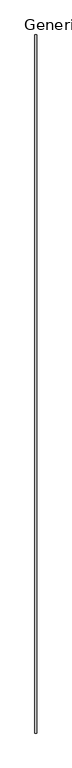
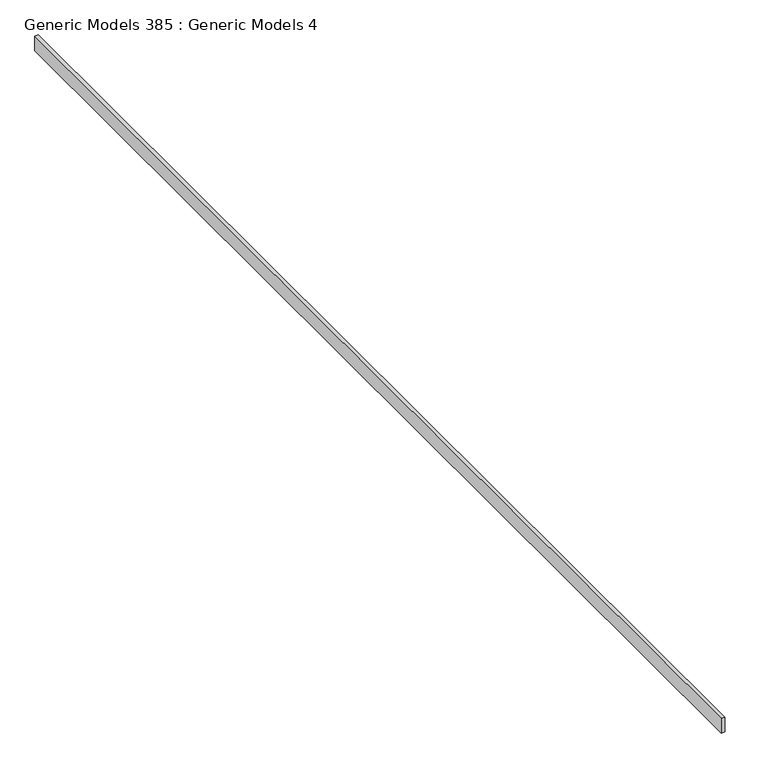
"""IFC4 building model written with IfcOpenShell, lengths in millimetres: proxy geometry, Generic Models 385 : Generic Models 4."""

import ifcopenshell
import ifcopenshell.guid

model = None  # the IFC model being written
_history = None  # IfcOwnerHistory: only IFC2X3 demands one
_inside = {}  # id of a spatial element -> (the spatial element, [elements in it])
_under = {}  # id of a project, library or spatial element -> (it, [spatial elements below it])
_declared = {}  # id of a project -> (the project, [libraries it declares])
_typed = {}  # id of a type object -> (the type object, [elements of that type])
_made_of = {}  # id of a material, layer set ... -> (it, [elements and type objects made of it])


def new_model(schema):
    """Start an empty IFC model of exactly this schema.

    Asked for "IFC4X3", IfcOpenShell would pick the latest addendum, in which some entities
    have other attributes; the version numbers below select the first issue.
    IFC2X3 requires an IfcOwnerHistory on every rooted entity: one is made here for all.
    """
    global model, _history
    if schema == "IFC4X3":
        model = ifcopenshell.file(schema_version=(4, 3, 0, 0))
    else:
        model = ifcopenshell.file(schema=schema)
    _inside.clear()
    _under.clear()
    _declared.clear()
    _typed.clear()
    _made_of.clear()
    _history = None
    if model.schema == "IFC2X3":
        org = make("IfcOrganization", Name="unknown")
        user = make(
            "IfcPersonAndOrganization",
            ThePerson=make("IfcPerson", FamilyName="unknown"),
            TheOrganization=org,
        )
        app = make(
            "IfcApplication",
            ApplicationDeveloper=org,
            Version="unknown",
            ApplicationFullName="unknown",
            ApplicationIdentifier="unknown",
        )
        _history = make(
            "IfcOwnerHistory",
            OwningUser=user,
            OwningApplication=app,
            ChangeAction="ADDED",
            CreationDate=0,
        )
    return model


def make(cls, **values):
    """One entity of the class cls with the attributes given. An attribute that is None is left unset."""
    return model.create_entity(
        cls, **{name: value for name, value in values.items() if value is not None}
    )


def rooted(cls, **values):
    """An entity with a GlobalId (a new one), such as an element, a storey or a relation."""
    return make(cls, GlobalId=ifcopenshell.guid.new(), OwnerHistory=_history, **values)


def si_unit(unit_type, name, prefix=None):
    """IfcSIUnit, for example si_unit("LENGTHUNIT", "METRE", prefix="MILLI")."""
    return make("IfcSIUnit", UnitType=unit_type, Prefix=prefix, Name=name)


def assignment(units):
    """IfcUnitAssignment: the units of a project."""
    return None if units is None else make("IfcUnitAssignment", Units=units)


def point(xyz):
    """IfcCartesianPoint."""
    return None if xyz is None else make("IfcCartesianPoint", Coordinates=xyz)


def direction(xyz):
    """IfcDirection."""
    return None if xyz is None else make("IfcDirection", DirectionRatios=xyz)


def frame(location, z_axis=None, x_axis=None):
    """IfcAxis2Placement3D, a coordinate frame: its origin and axes. An axis left out is left unset."""
    return make(
        "IfcAxis2Placement3D",
        Location=point(location),
        Axis=direction(z_axis),
        RefDirection=direction(x_axis),
    )


def origin():
    """The frame at (0, 0, 0) with its axes left unset."""
    return frame((0.0, 0.0, 0.0))


def place(relative_to, where):
    """IfcLocalPlacement: puts the frame where relative to a parent placement (None: the world)."""
    return make(
        "IfcLocalPlacement", PlacementRelTo=relative_to, RelativePlacement=where
    )


def context(
    kind, dimensions, precision=None, world=None, true_north=None, identifier=None
):
    """IfcGeometricRepresentationContext, for example the 3D "Model" context."""
    return make(
        "IfcGeometricRepresentationContext",
        ContextIdentifier=identifier,
        ContextType=kind,
        CoordinateSpaceDimension=dimensions,
        Precision=precision,
        WorldCoordinateSystem=world,
        TrueNorth=true_north,
    )


def project(units=None, contexts=None):
    """IfcProject with its units and contexts."""
    return rooted(
        "IfcProject",
        Name="project",
        RepresentationContexts=contexts,
        UnitsInContext=assignment(units),
    )


def spatial(cls, under=None, at=None, **own):
    """A site, building, storey or space (cls), placed at a placement, below another one or the project."""
    s = rooted(cls, ObjectPlacement=at, **own)
    if under is not None:
        _under.setdefault(under.id(), (under, []))[1].append(s)
    return s


def polyline(points):
    """IfcPolyline through the points."""
    return make("IfcPolyline", Points=[point(p) for p in points])


def outline(outer, holes=None, kind="AREA"):
    """IfcArbitraryClosedProfileDef: a profile drawn as a closed curve; with holes, ...WithVoids."""
    if holes is None:
        return make("IfcArbitraryClosedProfileDef", ProfileType=kind, OuterCurve=outer)
    return make(
        "IfcArbitraryProfileDefWithVoids",
        ProfileType=kind,
        OuterCurve=outer,
        InnerCurves=holes,
    )


def extrude(swept, where, along, depth):
    """IfcExtrudedAreaSolid: the profile swept, set in the frame where, extruded along a direction by depth."""
    return make(
        "IfcExtrudedAreaSolid",
        SweptArea=swept,
        Position=where,
        ExtrudedDirection=direction(along),
        Depth=depth,
    )


def shape(context_of_items, identifier, shape_type, items):
    """IfcShapeRepresentation: the items that make up one representation, for example the "Body"."""
    return make(
        "IfcShapeRepresentation",
        ContextOfItems=context_of_items,
        RepresentationIdentifier=identifier,
        RepresentationType=shape_type,
        Items=items,
    )


def source(mapping_origin, context_of_items, identifier, shape_type, items):
    """IfcRepresentationMap: a shape defined once, which mapped items show again and again."""
    return make(
        "IfcRepresentationMap",
        MappingOrigin=mapping_origin,
        MappedRepresentation=shape(context_of_items, identifier, shape_type, items),
    )


def transform(
    local_origin,
    x_axis=None,
    y_axis=None,
    z_axis=None,
    scale=None,
    scale2=None,
    scale3=None,
    uniform=True,
):
    """IfcCartesianTransformationOperator3D, or its non-uniform kind. x_axis, y_axis, z_axis: its Axis1, 2, 3."""
    if uniform:
        return make(
            "IfcCartesianTransformationOperator3D",
            Axis1=direction(x_axis),
            Axis2=direction(y_axis),
            LocalOrigin=point(local_origin),
            Scale=scale,
            Axis3=direction(z_axis),
        )
    return make(
        "IfcCartesianTransformationOperator3DnonUniform",
        Axis1=direction(x_axis),
        Axis2=direction(y_axis),
        LocalOrigin=point(local_origin),
        Scale=scale,
        Axis3=direction(z_axis),
        Scale2=scale2,
        Scale3=scale3,
    )


def mapped(mapping_source, mapping_target):
    """IfcMappedItem: shows the shape of a source again, moved by a transform."""
    return make(
        "IfcMappedItem", MappingSource=mapping_source, MappingTarget=mapping_target
    )


def made_of(thing, what):
    """Note that an element or type object is made of a material, layer set ...; save() writes the relation."""
    if what is not None:
        _made_of.setdefault(what.id(), (what, []))[1].append(thing)
    return thing


def element(
    cls,
    number,
    at=None,
    inside=None,
    cuts=None,
    type_object=None,
    material=None,
    context=None,
    identifier="Body",
    shape_type=None,
    held_by="IfcProductDefinitionShape",
    body=None,
    shapes=None,
    **own,
):
    """One element of the class cls, such as IfcWall. Its Tag is "e" and its number.

    at: its placement. inside: the storey or other place that contains it. cuts: it is an
    opening in that element (IfcRelVoidsElement). A single representation is given by context,
    identifier, shape_type and body (its items); several are given by shapes. held_by: the class
    of the entity that holds the representations. save() writes the other relations.
    """
    e = rooted(cls, Tag="e%d" % number, ObjectPlacement=at, **own)
    if body is not None:
        shapes = [shape(context, identifier, shape_type, body)]
    if shapes is not None:
        e.Representation = make(held_by, Representations=shapes)
    if inside is not None:
        _inside.setdefault(inside.id(), (inside, []))[1].append(e)
    if cuts is not None:
        rooted(
            "IfcRelVoidsElement", RelatingBuildingElement=cuts, RelatedOpeningElement=e
        )
    if type_object is not None:
        _typed.setdefault(type_object.id(), (type_object, []))[1].append(e)
    return made_of(e, material)


def aggregate(whole, parts):
    """IfcRelAggregates: a whole, such as a stair, and the parts it consists of."""
    return rooted("IfcRelAggregates", RelatingObject=whole, RelatedObjects=parts)


def save(model, path):
    """Write the relations noted so far, then the file.

    IfcRelAggregates (storeys below a building ...), IfcRelContainedInSpatialStructure (elements
    in a storey), IfcRelDefinesByType, IfcRelAssociatesMaterial and IfcRelDeclares: one each for
    every whole, place, type object, material and project.
    """
    for whole, parts in _under.values():
        aggregate(whole, parts)
    for where, things in _inside.values():
        rooted(
            "IfcRelContainedInSpatialStructure",
            RelatedElements=things,
            RelatingStructure=where,
        )
    for kind, things in _typed.values():
        rooted("IfcRelDefinesByType", RelatedObjects=things, RelatingType=kind)
    for what, things in _made_of.values():
        rooted("IfcRelAssociatesMaterial", RelatedObjects=things, RelatingMaterial=what)
    for by, libraries in _declared.values():
        rooted("IfcRelDeclares", RelatingContext=by, RelatedDefinitions=libraries)
    model.write(path)


def generic_models_385_generic_models_4_06af05cc(model_context):
    return source(origin(), model_context, "Body", "SweptSolid", [
        extrude(outline(polyline([(8346.0514146, -6864.9230338), (8327.0014146, -6864.9230338), (8327.0014146, -464.1230338), (8346.0514146, -464.1230338), (8346.0514146, -6864.9230338)])), frame((0.0, 0.0, 126250.2332283), z_axis=(0.0, 0.0, 1.0), x_axis=(1.0, 0.0, 0.0)), (0.0, 0.0, 1.0), 83.6072898),
    ])


if __name__ == "__main__":
    model = new_model("IFC4")
    model_context = context("Model", 3, world=origin())
    ifc_project = project(units=[si_unit("LENGTHUNIT", "METRE", prefix="MILLI")], contexts=[model_context])
    site = spatial("IfcSite", under=ifc_project)
    building = spatial("IfcBuilding", under=site)
    placement = place(None, origin())
    generic_models_385_generic_models_4_shape = generic_models_385_generic_models_4_06af05cc(model_context)
    element("IfcBuildingElementProxy", 1, Name="Generic Models 385 : Generic Models 4", ObjectType="Generic Models 385 : Generic Models 4", at=placement, inside=building, context=model_context, shape_type="MappedRepresentation", body=[
        mapped(generic_models_385_generic_models_4_shape, transform((0.0, 0.0, 0.0), x_axis=(1.0, 0.0, 0.0), y_axis=(0.0, 1.0, 0.0), z_axis=(0.0, 0.0, 1.0))),
    ])
    save(model, "model.ifc")

# Revit data of these elements
# Element 1 (IfcBuildingElementProxy, "Generic Models 385 : Generic Models 4")
#   Materials on its faces: "_CDX PLYWOOD - SEE STRUCT DWGs"
# Materials
#   "_CDX PLYWOOD - SEE STRUCT DWGs": class "Generic", colour RGB 98 75 74, transparency 0, Cost = 0
